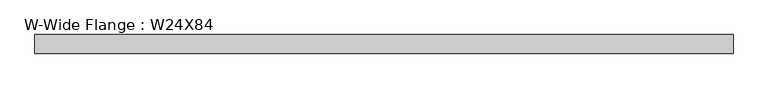
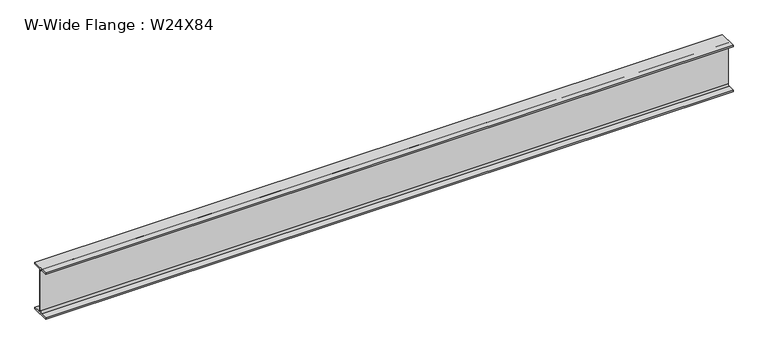
"""IFC4 building model written with IfcOpenShell, lengths in millimetres: beam geometry, W-Wide Flange : W24X84."""

from ifc_helpers import new_model, si_unit, point, frame, frame_2d, origin, place, context, project, spatial, polyline, circle_curve, trimmed, segment, composite_curve, outline, extrude, source, transform, mapped, element, save


def w_wide_flange_w24x84_97a9cff7(model_context):
    return source(origin(), model_context, "Body", "SweptSolid", [
        extrude(outline(composite_curve([segment(polyline([(114.554, -286.512), (114.554, -306.07), (-114.554, -306.07), (-114.554, -286.512), (-29.2735, -286.512)]), True, "CONTINUOUS"), segment(trimmed(circle_curve(frame_2d((-29.2735, -263.2075)), 23.3045), [point((-29.2735, -286.512))], [point((-5.969, -263.2075))], True, "CARTESIAN"), True, "CONTINUOUS"), segment(polyline([(-5.969, -263.2075), (-5.969, 263.2075)]), True, "CONTINUOUS"), segment(trimmed(circle_curve(frame_2d((-29.2735, 263.2075)), 23.3045), [point((-5.969, 263.2075))], [point((-29.2735, 286.512))], True, "CARTESIAN"), True, "CONTINUOUS"), segment(polyline([(-29.2735, 286.512), (-114.554, 286.512), (-114.554, 306.07), (114.554, 306.07), (114.554, 286.512), (29.2735, 286.512)]), True, "CONTINUOUS"), segment(trimmed(circle_curve(frame_2d((29.2735, 263.2075)), 23.3045), [point((29.2735, 286.512))], [point((5.969, 263.2075))], True, "CARTESIAN"), True, "CONTINUOUS"), segment(polyline([(5.969, 263.2075), (5.969, -263.2075)]), True, "CONTINUOUS"), segment(trimmed(circle_curve(frame_2d((29.2735, -263.2075)), 23.3045), [point((5.969, -263.2075))], [point((29.2735, -286.512))], True, "CARTESIAN"), True, "CONTINUOUS"), segment(polyline([(29.2735, -286.512), (114.554, -286.512)]), True, "CONTINUOUS")], self_intersect=False)), frame((-4221.1128906, 0.0, 0.0), z_axis=(1.0, 0.0, 0.0), x_axis=(0.0, 1.0, 0.0)), (0.0, 0.0, 1.0), 8577.1632812),
    ])


if __name__ == "__main__":
    model = new_model("IFC4")
    model_context = context("Model", 3, world=origin())
    ifc_project = project(units=[si_unit("LENGTHUNIT", "METRE", prefix="MILLI")], contexts=[model_context])
    site = spatial("IfcSite", under=ifc_project)
    building = spatial("IfcBuilding", under=site)
    placement = place(None, origin())
    w_wide_flange_w24x84_shape = w_wide_flange_w24x84_97a9cff7(model_context)
    element("IfcBeam", 1, ObjectType="W-Wide Flange : W24X84", at=placement, inside=building, context=model_context, shape_type="MappedRepresentation", body=[
        mapped(w_wide_flange_w24x84_shape, transform((0.0, 0.0, 0.0), x_axis=(1.0, 0.0, 0.0), y_axis=(0.0, 1.0, 0.0), z_axis=(0.0, 0.0, 1.0))),
    ])
    save(model, "model.ifc")

# Revit data of these elements
# Type "W-Wide Flange : W24X84"
#   Assembly Code = "B10"
#   W = 84
#   Length [instance default] = 1524 mm
#   bf = 229.108 mm
#   d = 612.14 mm
#   k = 42.863 mm
#   k2 = 23.305 mm
#   tf = 19.558 mm
#   tw = 11.938 mm
#   A = 0.0159355 m²
#   Structural Material [instance default] = Steel ASTM A992
# Element 1 (IfcBeam, "W-Wide Flange : W24X84")
#   Structural Material = Aluminum, Anodized Red
#   Materials on its faces: "Aluminum, Anodized Red"
# Materials
#   "Steel ASTM A992": class "Metal", colour RGB 128 0 0, transparency 0, Description = "Structural steel 50ksi", Cost = 0
#   "Aluminum, Anodized Red": class "Metal", colour RGB 120 120 120, transparency 0, Description = "Anodized aluminum, red", Cost = 0
